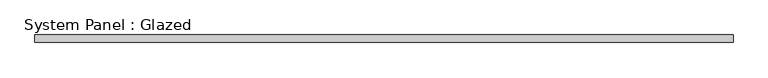
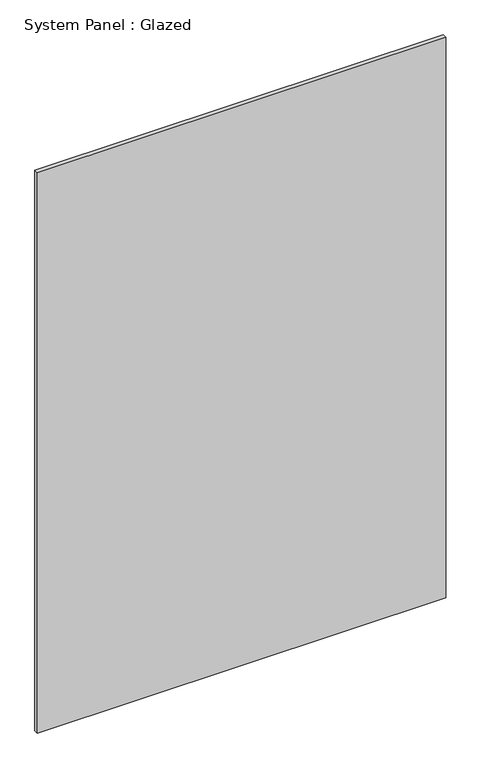
"""IFC4 building model written with IfcOpenShell, lengths in millimetres: plate geometry, System Panel : Glazed."""

from ifc_helpers import new_model, si_unit, origin, origin_with_axes, place, context, project, spatial, polyline, outline, extrude, source, transform, mapped, element, save


def system_panel_glazed_6ba5d601(model_context):
    return source(origin(), model_context, "Body", "SweptSolid", [
        extrude(outline(polyline([(1161.571127, 24.5), (-1161.571127, 24.5), (-1161.571127, 49.5), (1161.571127, 49.5), (1161.571127, 24.5)])), origin_with_axes(), (0.0, 0.0, 1.0), 3370.0),
    ])


if __name__ == "__main__":
    model = new_model("IFC4")
    model_context = context("Model", 3, world=origin())
    ifc_project = project(units=[si_unit("LENGTHUNIT", "METRE", prefix="MILLI")], contexts=[model_context])
    site = spatial("IfcSite", under=ifc_project)
    building = spatial("IfcBuilding", under=site)
    placement = place(None, origin())
    system_panel_glazed_shape = system_panel_glazed_6ba5d601(model_context)
    element("IfcPlate", 1, ObjectType="System Panel : Glazed", at=placement, inside=building, context=model_context, shape_type="MappedRepresentation", body=[
        mapped(system_panel_glazed_shape, transform((0.0, 0.0, 0.0), x_axis=(1.0, 0.0, 0.0), y_axis=(0.0, 1.0, 0.0), z_axis=(0.0, 0.0, 1.0))),
    ])
    save(model, "model.ifc")

# Revit data of these elements
# Type "System Panel : Glazed"
#   Construction Type Id = "GSP4R"
#   Analytic Construction = "1/8 in Pilkington single glazing"
#   Visual Light Transmittance = 0.9
#   Solar Heat Gain Coefficient = 0.86
#   Heat Transfer Coefficient (U) = 6.7069 W/(m²·K)
#   Define Thermal Properties by = 1
# Element 1 (IfcPlate, "System Panel : Glazed")
#   Materials on its faces: "Glass"
# Materials
#   "Glass": class "Glass", colour RGB 245 245 243, transparency 1, Description = "Soda Lime Glass", Cost = 0
